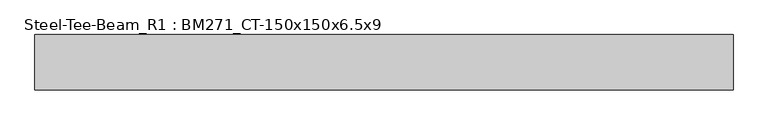
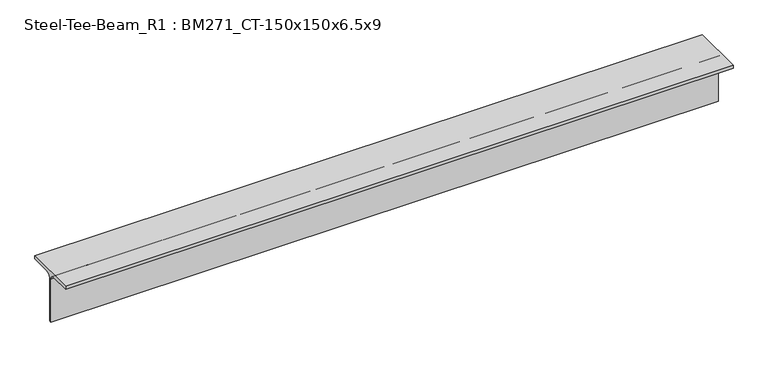
"""IFC4 building model written with IfcOpenShell, lengths in millimetres: member geometry, Steel-Tee-Beam_R1 : BM271_CT-150x150x6.5x9."""

from ifc_helpers import new_model, si_unit, point, frame, frame_2d, origin, place, context, project, spatial, polyline, circle_curve, trimmed, segment, composite_curve, outline, extrude, source, transform, mapped, element, save


def steel_tee_beam_r1_bm271_ct_150x150x6_5x9_2e8d7a99(model_context):
    return source(origin(), model_context, "Body", "SweptSolid", [
        extrude(outline(composite_curve([segment(polyline([(75.0, 75.0), (75.0, 66.0), (16.25, 66.0)]), True, "CONTINUOUS"), segment(trimmed(circle_curve(frame_2d((16.25, 53.0)), 13.0), [point((16.25, 66.0))], [point((3.25, 53.0))], True, "CARTESIAN"), True, "CONTINUOUS"), segment(polyline([(3.25, 53.0), (3.25, -75.0), (-3.25, -75.0), (-3.25, 53.0)]), True, "CONTINUOUS"), segment(trimmed(circle_curve(frame_2d((-16.25, 53.0)), 13.0), [point((-3.25, 53.0))], [point((-16.25, 66.0))], True, "CARTESIAN"), True, "CONTINUOUS"), segment(polyline([(-16.25, 66.0), (-75.0, 66.0), (-75.0, 75.0), (75.0, 75.0)]), True, "CONTINUOUS")], self_intersect=False)), frame((-900.1288904, 0.0, 0.0), z_axis=(1.0, 0.0, 0.0), x_axis=(0.0, 1.0, 0.0)), (0.0, 0.0, 1.0), 1884.11033),
    ])


if __name__ == "__main__":
    model = new_model("IFC4")
    model_context = context("Model", 3, world=origin())
    ifc_project = project(units=[si_unit("LENGTHUNIT", "METRE", prefix="MILLI")], contexts=[model_context])
    site = spatial("IfcSite", under=ifc_project)
    building = spatial("IfcBuilding", under=site)
    placement = place(None, origin())
    steel_tee_beam_r1_bm271_ct_150x150x6_5x9_shape = steel_tee_beam_r1_bm271_ct_150x150x6_5x9_2e8d7a99(model_context)
    element("IfcMember", 1, ObjectType="Steel-Tee-Beam_R1 : BM271_CT-150x150x6.5x9", at=placement, inside=building, context=model_context, shape_type="MappedRepresentation", body=[
        mapped(steel_tee_beam_r1_bm271_ct_150x150x6_5x9_shape, transform((0.0, 0.0, 0.0), x_axis=(1.0, 0.0, 0.0), y_axis=(0.0, 1.0, 0.0), z_axis=(0.0, 0.0, 1.0))),
    ])
    save(model, "model.ifc")

# Revit data of these elements
# Type "Steel-Tee-Beam_R1 : BM271_CT-150x150x6.5x9"
#   Keynote = "CT-150x150x6.5x9"
#   Surface Area = 0.588841 m²/m
#   Section Area = 23.3904 cm²
#   Mass per Unit Length = 18.3614 kg/m
#   Length [instance default] = 1.5240 m
#   bf = 0.1500 m
#   d = 0.1500 m
#   k = 0.0220 m
#   r = 0.0130 m
#   tf = 0.0090 m
#   tw = 0.0065 m
#   hec_material4 [instance default] = none
#   hec_material3 [instance default] = none
#   hec_material2 [instance default] = none
#   hec_material1 [instance default] = none
#   Structural Material [instance default] = Steel, 45-345
#   Assembly Code = ""
# Element 1 (IfcMember, "Steel-Tee-Beam_R1 : BM271_CT-150x150x6.5x9")
#   Structural Material = none
# Materials
#   "Steel, 45-345": class "Metal", colour RGB 189 187 185, transparency 0, Description = "Steel 345 MPa", Cost = 0
